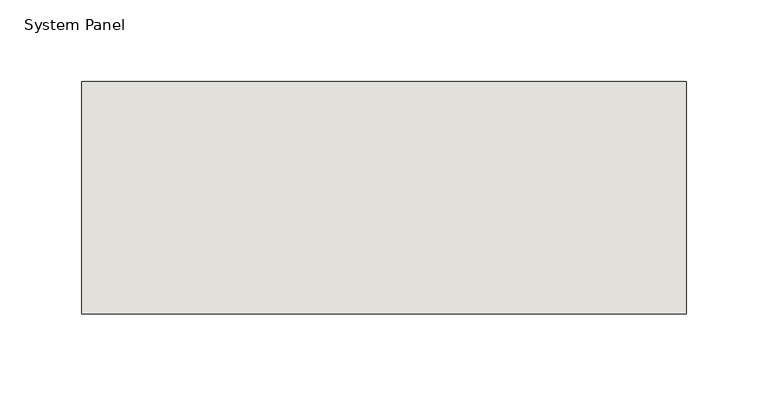
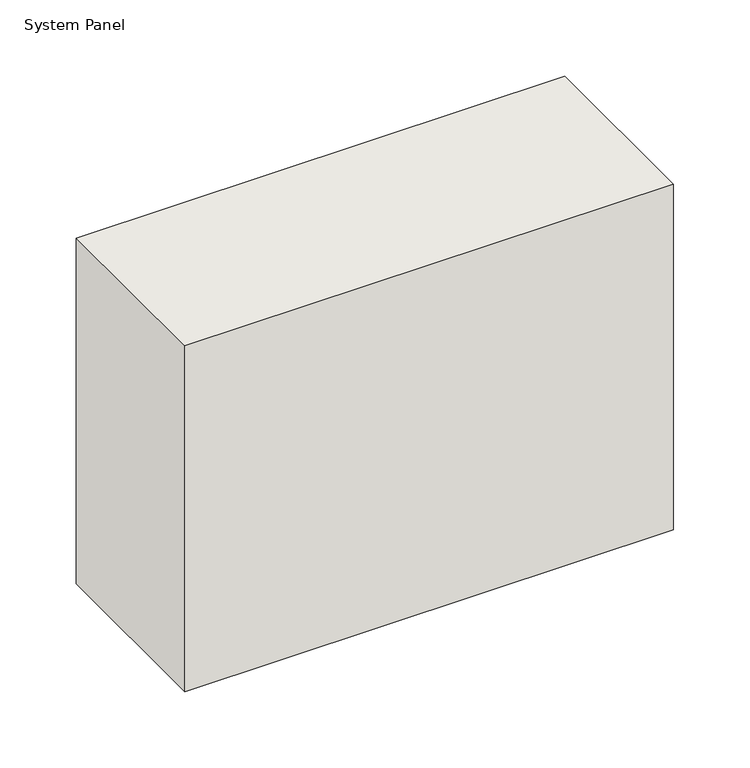
"""IFC4 building model written with IfcOpenShell, lengths in millimetres: wall geometry, System Panel : NLRS_21_CWP_hsb-vulling minerale wol 142 _gen_rsf."""

from ifc_helpers import new_model, si_unit, origin, origin_with_axes, place, context, project, spatial, polyline, outline, extrude, source, transform, mapped, element, save


def system_panel_0d6cc1c8(model_context):
    return source(origin(), model_context, "Body", "SweptSolid", [
        extrude(outline(polyline([(184.5, -71.0), (-184.5, -71.0), (-184.5, 71.0), (184.5, 71.0), (184.5, -71.0)])), origin_with_axes(), (0.0, 0.0, 1.0), 276.0),
    ])


if __name__ == "__main__":
    model = new_model("IFC4")
    model_context = context("Model", 3, world=origin())
    ifc_project = project(units=[si_unit("LENGTHUNIT", "METRE", prefix="MILLI")], contexts=[model_context])
    site = spatial("IfcSite", under=ifc_project)
    building = spatial("IfcBuilding", under=site)
    placement = place(None, origin())
    system_panel_shape = system_panel_0d6cc1c8(model_context)
    element("IfcWall", 1, ObjectType="System Panel : NLRS_21_CWP_hsb-vulling minerale wol 142 _gen_rsf", at=placement, inside=building, context=model_context, shape_type="MappedRepresentation", body=[
        mapped(system_panel_shape, transform((0.0, 0.0, 0.0), x_axis=(1.0, 0.0, 0.0), y_axis=(0.0, 1.0, 0.0), z_axis=(0.0, 0.0, 1.0))),
    ])
    save(model, "model.ifc")

# Revit data of these elements
# Type "System Panel : NLRS_21_CWP_hsb-vulling minerale wol 142 _gen_rsf"
#   Type IfcGUID = "07M7mRoiH1CR8m_RSKIwpC"
#   Assembly Code = "21.23"
#   IfcExportAs = "IfcWall"
# Element 1 (IfcWall, "System Panel : NLRS_21_CWP_hsb-vulling minerale wol 142 _gen_rsf")
#   Materials on its faces: "NLRS_m1_isolatie minerale wol_gen_rsf"
# Materials
#   "NLRS_m1_isolatie minerale wol_gen_rsf": class "M - Anorganische materialen", colour RGB 200 200 140, transparency 0, Keynote = "m1", Manufacturer = "Revit Standards Foundation", URL = "www.revitstandards.org", Description = "isolatie minerale wol", Cost = 0
